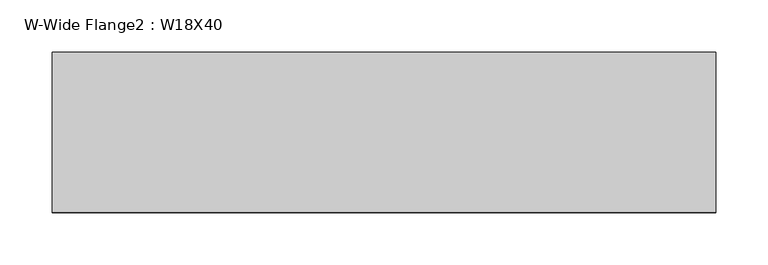
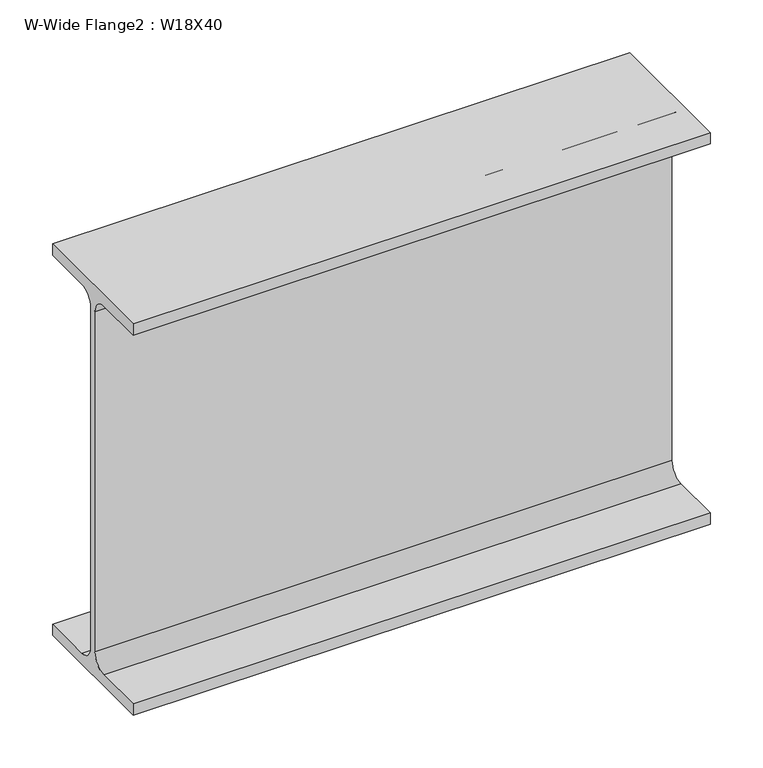
"""IFC4 building model written with IfcOpenShell, lengths in millimetres: beam geometry, W-Wide Flange2 : W18X40."""

from ifc_helpers import new_model, si_unit, point, frame, frame_2d, origin, place, context, project, spatial, polyline, circle_curve, trimmed, segment, composite_curve, outline, extrude, source, transform, mapped, element, save


def w_wide_flange2_w18x40_85773016(model_context):
    return source(origin(), model_context, "Body", "SweptSolid", [
        extrude(outline(composite_curve([segment(polyline([(76.454, -213.995), (76.454, -227.33), (-76.454, -227.33), (-76.454, -213.995), (-20.828, -213.995)]), True, "CONTINUOUS"), segment(trimmed(circle_curve(frame_2d((-20.828, -197.1675)), 16.8275), [point((-20.828, -213.995))], [point((-4.0005, -197.1675))], True, "CARTESIAN"), True, "CONTINUOUS"), segment(polyline([(-4.0005, -197.1675), (-4.0005, 197.1675)]), True, "CONTINUOUS"), segment(trimmed(circle_curve(frame_2d((-20.828, 197.1675)), 16.8275), [point((-4.0005, 197.1675))], [point((-20.828, 213.995))], True, "CARTESIAN"), True, "CONTINUOUS"), segment(polyline([(-20.828, 213.995), (-76.454, 213.995), (-76.454, 227.33), (76.454, 227.33), (76.454, 213.995), (20.828, 213.995)]), True, "CONTINUOUS"), segment(trimmed(circle_curve(frame_2d((20.828, 197.1675)), 16.8275), [point((20.828, 213.995))], [point((4.0005, 197.1675))], True, "CARTESIAN"), True, "CONTINUOUS"), segment(polyline([(4.0005, 197.1675), (4.0005, -197.1675)]), True, "CONTINUOUS"), segment(trimmed(circle_curve(frame_2d((20.828, -197.1675)), 16.8275), [point((4.0005, -197.1675))], [point((20.828, -213.995))], True, "CARTESIAN"), True, "CONTINUOUS"), segment(polyline([(20.828, -213.995), (76.454, -213.995)]), True, "CONTINUOUS")], self_intersect=False)), frame((-345.28125, 0.0, 0.0), z_axis=(1.0, 0.0, 0.0), x_axis=(0.0, 1.0, 0.0)), (0.0, 0.0, 1.0), 633.4125),
    ])


if __name__ == "__main__":
    model = new_model("IFC4")
    model_context = context("Model", 3, world=origin())
    ifc_project = project(units=[si_unit("LENGTHUNIT", "METRE", prefix="MILLI")], contexts=[model_context])
    site = spatial("IfcSite", under=ifc_project)
    building = spatial("IfcBuilding", under=site)
    placement = place(None, origin())
    w_wide_flange2_w18x40_shape = w_wide_flange2_w18x40_85773016(model_context)
    element("IfcBeam", 1, ObjectType="W-Wide Flange2 : W18X40", at=placement, inside=building, context=model_context, shape_type="MappedRepresentation", body=[
        mapped(w_wide_flange2_w18x40_shape, transform((0.0, 0.0, 0.0), x_axis=(1.0, 0.0, 0.0), y_axis=(0.0, 1.0, 0.0), z_axis=(0.0, 0.0, 1.0))),
    ])
    save(model, "model.ifc")

# Revit data of these elements
# Type "W-Wide Flange2 : W18X40"
#   Assembly Code = "B10"
#   W = 40
#   Length [instance default] = 5' - 0"
#   bf = 0' - 6.02"
#   d = 1' - 5.9"
#   k = 0' - 1 3/16"
#   k2 = 0' - 0.6625"
#   tf = 0' - 0.525"
#   tw = 0' - 0.315"
#   A = 0.0819444 SF
#   Structural Material [instance default] = Steel ASTM A992
# Element 1 (IfcBeam, "W-Wide Flange2 : W18X40")
#   Materials on its faces: "Steel ASTM A992"
# Materials
#   "Steel ASTM A992": class "Metal", colour RGB 199 199 199, transparency 0, Description = "Structural steel 50ksi", Cost = 0
